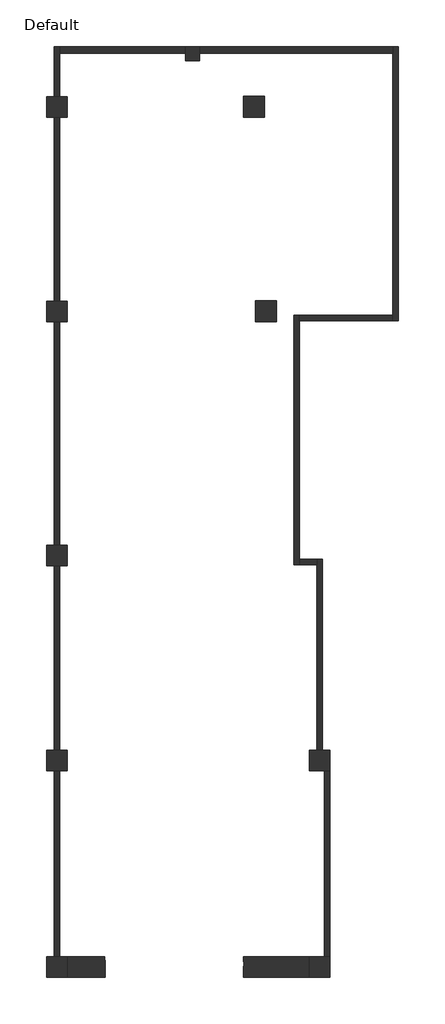
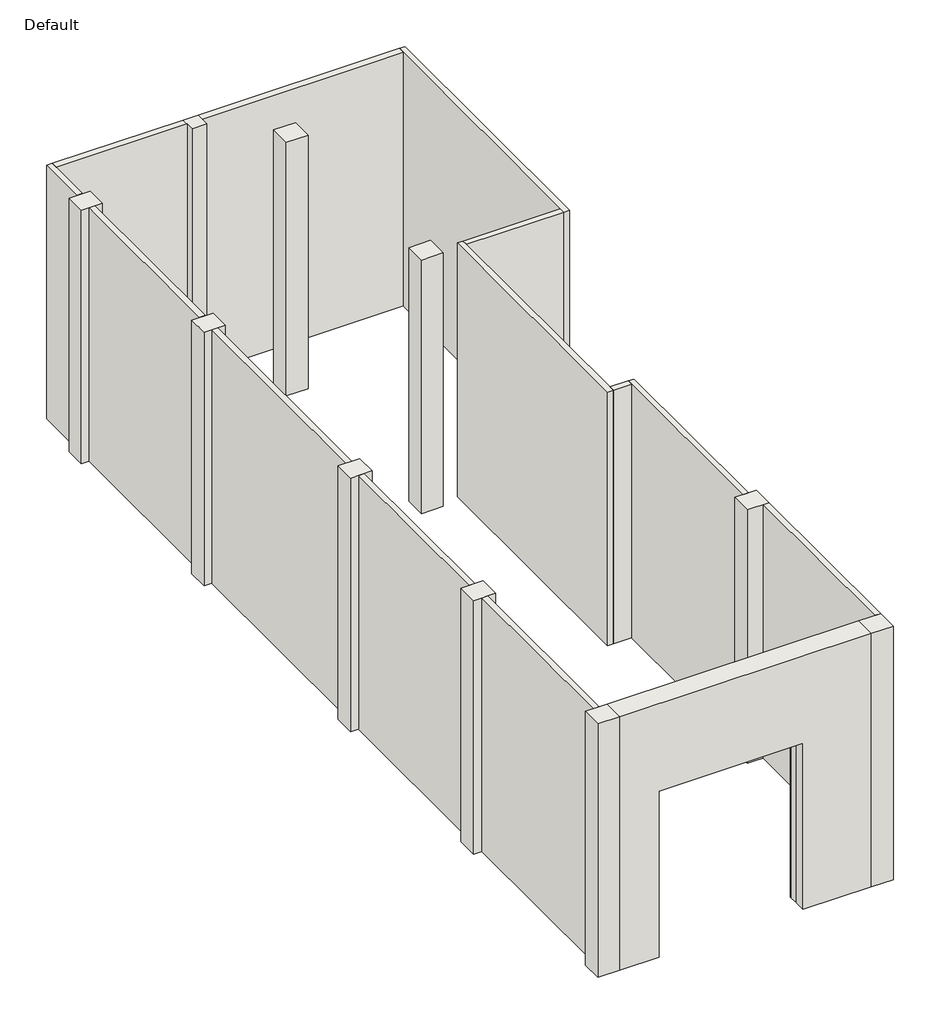
# One storey: 24 walls.
"""IFC4 building model written with IfcOpenShell, lengths in millimetres."""

import ifcopenshell
import ifcopenshell.guid

model = None  # the IFC model being written
_history = None  # IfcOwnerHistory: only IFC2X3 demands one
_inside = {}  # id of a spatial element -> (the spatial element, [elements in it])
_under = {}  # id of a project, library or spatial element -> (it, [spatial elements below it])
_declared = {}  # id of a project -> (the project, [libraries it declares])
_typed = {}  # id of a type object -> (the type object, [elements of that type])
_made_of = {}  # id of a material, layer set ... -> (it, [elements and type objects made of it])


def new_model(schema):
    """Start an empty IFC model of exactly this schema.

    Asked for "IFC4X3", IfcOpenShell would pick the latest addendum, in which some entities
    have other attributes; the version numbers below select the first issue.
    IFC2X3 requires an IfcOwnerHistory on every rooted entity: one is made here for all.
    """
    global model, _history
    if schema == "IFC4X3":
        model = ifcopenshell.file(schema_version=(4, 3, 0, 0))
    else:
        model = ifcopenshell.file(schema=schema)
    _inside.clear()
    _under.clear()
    _declared.clear()
    _typed.clear()
    _made_of.clear()
    _history = None
    if model.schema == "IFC2X3":
        org = make("IfcOrganization", Name="unknown")
        user = make(
            "IfcPersonAndOrganization",
            ThePerson=make("IfcPerson", FamilyName="unknown"),
            TheOrganization=org,
        )
        app = make(
            "IfcApplication",
            ApplicationDeveloper=org,
            Version="unknown",
            ApplicationFullName="unknown",
            ApplicationIdentifier="unknown",
        )
        _history = make(
            "IfcOwnerHistory",
            OwningUser=user,
            OwningApplication=app,
            ChangeAction="ADDED",
            CreationDate=0,
        )
    return model


def make(cls, **values):
    """One entity of the class cls with the attributes given. An attribute that is None is left unset."""
    return model.create_entity(
        cls, **{name: value for name, value in values.items() if value is not None}
    )


def rooted(cls, **values):
    """An entity with a GlobalId (a new one), such as an element, a storey or a relation."""
    return make(cls, GlobalId=ifcopenshell.guid.new(), OwnerHistory=_history, **values)


def si_unit(unit_type, name, prefix=None):
    """IfcSIUnit, for example si_unit("LENGTHUNIT", "METRE", prefix="MILLI")."""
    return make("IfcSIUnit", UnitType=unit_type, Prefix=prefix, Name=name)


def assignment(units):
    """IfcUnitAssignment: the units of a project."""
    return None if units is None else make("IfcUnitAssignment", Units=units)


def point(xyz):
    """IfcCartesianPoint."""
    return None if xyz is None else make("IfcCartesianPoint", Coordinates=xyz)


def direction(xyz):
    """IfcDirection."""
    return None if xyz is None else make("IfcDirection", DirectionRatios=xyz)


def frame(location, z_axis=None, x_axis=None):
    """IfcAxis2Placement3D, a coordinate frame: its origin and axes. An axis left out is left unset."""
    return make(
        "IfcAxis2Placement3D",
        Location=point(location),
        Axis=direction(z_axis),
        RefDirection=direction(x_axis),
    )


def origin():
    """The frame at (0, 0, 0) with its axes left unset."""
    return frame((0.0, 0.0, 0.0))


def origin_with_axes():
    """The frame at (0, 0, 0) with the z axis (0, 0, 1) and the x axis (1, 0, 0) written out."""
    return frame((0.0, 0.0, 0.0), z_axis=(0.0, 0.0, 1.0), x_axis=(1.0, 0.0, 0.0))


def place(relative_to, where):
    """IfcLocalPlacement: puts the frame where relative to a parent placement (None: the world)."""
    return make(
        "IfcLocalPlacement", PlacementRelTo=relative_to, RelativePlacement=where
    )


def context(
    kind, dimensions, precision=None, world=None, true_north=None, identifier=None
):
    """IfcGeometricRepresentationContext, for example the 3D "Model" context."""
    return make(
        "IfcGeometricRepresentationContext",
        ContextIdentifier=identifier,
        ContextType=kind,
        CoordinateSpaceDimension=dimensions,
        Precision=precision,
        WorldCoordinateSystem=world,
        TrueNorth=true_north,
    )


def project(units=None, contexts=None):
    """IfcProject with its units and contexts."""
    return rooted(
        "IfcProject",
        Name="project",
        RepresentationContexts=contexts,
        UnitsInContext=assignment(units),
    )


def spatial(cls, under=None, at=None, **own):
    """A site, building, storey or space (cls), placed at a placement, below another one or the project."""
    s = rooted(cls, ObjectPlacement=at, **own)
    if under is not None:
        _under.setdefault(under.id(), (under, []))[1].append(s)
    return s


def polyline(points):
    """IfcPolyline through the points."""
    return make("IfcPolyline", Points=[point(p) for p in points])


def outline(outer, holes=None, kind="AREA"):
    """IfcArbitraryClosedProfileDef: a profile drawn as a closed curve; with holes, ...WithVoids."""
    if holes is None:
        return make("IfcArbitraryClosedProfileDef", ProfileType=kind, OuterCurve=outer)
    return make(
        "IfcArbitraryProfileDefWithVoids",
        ProfileType=kind,
        OuterCurve=outer,
        InnerCurves=holes,
    )


def extrude(swept, where, along, depth):
    """IfcExtrudedAreaSolid: the profile swept, set in the frame where, extruded along a direction by depth."""
    return make(
        "IfcExtrudedAreaSolid",
        SweptArea=swept,
        Position=where,
        ExtrudedDirection=direction(along),
        Depth=depth,
    )


def faces_of(points, faces, orient=None, outer=None):
    """IfcFace entities. A face is a list of loops; a loop is a list of indices into points, from 0.

    orient and outer hold one flag for each loop. By default every Orientation is true, the
    first loop of a face is its IfcFaceOuterBound and the others are IfcFaceBound.
    """
    made = []
    for i, loops in enumerate(faces):
        bounds = []
        for j, loop in enumerate(loops):
            is_outer = j == 0 if outer is None else outer[i][j]
            bounds.append(
                make(
                    "IfcFaceOuterBound" if is_outer else "IfcFaceBound",
                    Bound=make("IfcPolyLoop", Polygon=[points[k] for k in loop]),
                    Orientation=True if orient is None else orient[i][j],
                )
            )
        made.append(make("IfcFace", Bounds=bounds))
    return made


def faceted_brep(points, faces, orient=None, outer=None, voids=None):
    """IfcFacetedBrep: a solid bounded by flat faces; with voids (closed shells), ...WithVoids."""
    shared = [point(p) for p in points]
    hull = make("IfcClosedShell", CfsFaces=faces_of(shared, faces, orient, outer))
    if voids is None:
        return make("IfcFacetedBrep", Outer=hull)
    return make(
        "IfcFacetedBrepWithVoids",
        Outer=hull,
        Voids=[
            make(cls, CfsFaces=faces_of(shared, fs, o, b)) for cls, fs, o, b in voids
        ],
    )


def shape(context_of_items, identifier, shape_type, items):
    """IfcShapeRepresentation: the items that make up one representation, for example the "Body"."""
    return make(
        "IfcShapeRepresentation",
        ContextOfItems=context_of_items,
        RepresentationIdentifier=identifier,
        RepresentationType=shape_type,
        Items=items,
    )


def source(mapping_origin, context_of_items, identifier, shape_type, items):
    """IfcRepresentationMap: a shape defined once, which mapped items show again and again."""
    return make(
        "IfcRepresentationMap",
        MappingOrigin=mapping_origin,
        MappedRepresentation=shape(context_of_items, identifier, shape_type, items),
    )


def transform(
    local_origin,
    x_axis=None,
    y_axis=None,
    z_axis=None,
    scale=None,
    scale2=None,
    scale3=None,
    uniform=True,
):
    """IfcCartesianTransformationOperator3D, or its non-uniform kind. x_axis, y_axis, z_axis: its Axis1, 2, 3."""
    if uniform:
        return make(
            "IfcCartesianTransformationOperator3D",
            Axis1=direction(x_axis),
            Axis2=direction(y_axis),
            LocalOrigin=point(local_origin),
            Scale=scale,
            Axis3=direction(z_axis),
        )
    return make(
        "IfcCartesianTransformationOperator3DnonUniform",
        Axis1=direction(x_axis),
        Axis2=direction(y_axis),
        LocalOrigin=point(local_origin),
        Scale=scale,
        Axis3=direction(z_axis),
        Scale2=scale2,
        Scale3=scale3,
    )


def mapped(mapping_source, mapping_target):
    """IfcMappedItem: shows the shape of a source again, moved by a transform."""
    return make(
        "IfcMappedItem", MappingSource=mapping_source, MappingTarget=mapping_target
    )


def made_of(thing, what):
    """Note that an element or type object is made of a material, layer set ...; save() writes the relation."""
    if what is not None:
        _made_of.setdefault(what.id(), (what, []))[1].append(thing)
    return thing


def element(
    cls,
    number,
    at=None,
    inside=None,
    cuts=None,
    type_object=None,
    material=None,
    context=None,
    identifier="Body",
    shape_type=None,
    held_by="IfcProductDefinitionShape",
    body=None,
    shapes=None,
    **own,
):
    """One element of the class cls, such as IfcWall. Its Tag is "e" and its number.

    at: its placement. inside: the storey or other place that contains it. cuts: it is an
    opening in that element (IfcRelVoidsElement). A single representation is given by context,
    identifier, shape_type and body (its items); several are given by shapes. held_by: the class
    of the entity that holds the representations. save() writes the other relations.
    """
    e = rooted(cls, Tag="e%d" % number, ObjectPlacement=at, **own)
    if body is not None:
        shapes = [shape(context, identifier, shape_type, body)]
    if shapes is not None:
        e.Representation = make(held_by, Representations=shapes)
    if inside is not None:
        _inside.setdefault(inside.id(), (inside, []))[1].append(e)
    if cuts is not None:
        rooted(
            "IfcRelVoidsElement", RelatingBuildingElement=cuts, RelatedOpeningElement=e
        )
    if type_object is not None:
        _typed.setdefault(type_object.id(), (type_object, []))[1].append(e)
    return made_of(e, material)


def aggregate(whole, parts):
    """IfcRelAggregates: a whole, such as a stair, and the parts it consists of."""
    return rooted("IfcRelAggregates", RelatingObject=whole, RelatedObjects=parts)


def save(model, path):
    """Write the relations noted so far, then the file.

    IfcRelAggregates (storeys below a building ...), IfcRelContainedInSpatialStructure (elements
    in a storey), IfcRelDefinesByType, IfcRelAssociatesMaterial and IfcRelDeclares: one each for
    every whole, place, type object, material and project.
    """
    for whole, parts in _under.values():
        aggregate(whole, parts)
    for where, things in _inside.values():
        rooted(
            "IfcRelContainedInSpatialStructure",
            RelatedElements=things,
            RelatingStructure=where,
        )
    for kind, things in _typed.values():
        rooted("IfcRelDefinesByType", RelatedObjects=things, RelatingType=kind)
    for what, things in _made_of.values():
        rooted("IfcRelAssociatesMaterial", RelatedObjects=things, RelatingMaterial=what)
    for by, libraries in _declared.values():
        rooted("IfcRelDeclares", RelatingContext=by, RelatedDefinitions=libraries)
    model.write(path)


def pillar_1_pillar_1_f30ecb4e(model_context):
    return source(origin(), model_context, "Body", "SweptSolid", [
        extrude(outline(polyline([(240.0, 0.0), (-140.0, 0.0), (-140.0, 380.0), (240.0, 380.0), (240.0, 0.0)])), origin_with_axes(), (0.0, 0.0, 1.0), 4700.0),
    ])


def pillar_10_pillar_10_9a1170d5(model_context):
    return source(origin(), model_context, "Body", "SweptSolid", [
        extrude(outline(polyline([(5040.0, 0.0), (4660.0, 0.0), (4660.0, 380.0), (5040.0, 380.0), (5040.0, 0.0)])), origin_with_axes(), (0.0, 0.0, 1.0), 4700.0),
    ])


def pillar_2_pillar_2_c342d97b(model_context):
    return source(origin(), model_context, "Body", "SweptSolid", [
        extrude(outline(polyline([(240.0, 3770.0), (-140.0, 3770.0), (-140.0, 4150.0), (240.0, 4150.0), (240.0, 3770.0)])), origin_with_axes(), (0.0, 0.0, 1.0), 4700.0),
    ])


def pillar_3_pillar_3_bef34371(model_context):
    return source(origin(), model_context, "Body", "SweptSolid", [
        extrude(outline(polyline([(240.0, 7510.0), (-140.0, 7510.0), (-140.0, 7890.0), (240.0, 7890.0), (240.0, 7510.0)])), origin_with_axes(), (0.0, 0.0, 1.0), 4700.0),
    ])


def pillar_4_pillar_4_1424975a(model_context):
    return source(origin(), model_context, "Body", "SweptSolid", [
        extrude(outline(polyline([(235.0, 11970.0), (-135.0, 11970.0), (-135.0, 12340.0), (235.0, 12340.0), (235.0, 11970.0)])), origin_with_axes(), (0.0, 0.0, 1.0), 4700.0),
    ])


def pillar_5_pillar_5_5ba1b83c(model_context):
    return source(origin(), model_context, "Body", "SweptSolid", [
        extrude(outline(polyline([(235.0, 15700.0), (-135.0, 15700.0), (-135.0, 16070.0), (235.0, 16070.0), (235.0, 15700.0)])), origin_with_axes(), (0.0, 0.0, 1.0), 4700.0),
    ])


def pillar_6_pillar_6_704e6477(model_context):
    return source(origin(), model_context, "Body", "SweptSolid", [
        extrude(outline(polyline([(2660.0, 16730.0), (2400.0, 16730.0), (2400.0, 16990.0), (2660.0, 16990.0), (2660.0, 16730.0)])), origin_with_axes(), (0.0, 0.0, 1.0), 4700.0),
    ])


def pillar_7_pillar_7_9e6fd231(model_context):
    return source(origin(), model_context, "Body", "SweptSolid", [
        extrude(outline(polyline([(3840.0, 15700.0), (3460.0, 15700.0), (3460.0, 16080.0), (3840.0, 16080.0), (3840.0, 15700.0)])), origin_with_axes(), (0.0, 0.0, 1.0), 4700.0),
    ])


def pillar_8_pillar_8_cf5ea2e7(model_context):
    return source(origin(), model_context, "Body", "SweptSolid", [
        extrude(outline(polyline([(4060.0, 11970.0), (3680.0, 11970.0), (3680.0, 12350.0), (4060.0, 12350.0), (4060.0, 11970.0)])), origin_with_axes(), (0.0, 0.0, 1.0), 4700.0),
    ])


def pillar_9_pillar_9_1ccd6465(model_context):
    return source(origin(), model_context, "Body", "SweptSolid", [
        extrude(outline(polyline([(5040.0, 3770.0), (4660.0, 3770.0), (4660.0, 4150.0), (5040.0, 4150.0), (5040.0, 3770.0)])), origin_with_axes(), (0.0, 0.0, 1.0), 4700.0),
    ])


def wall_1_wall_1_841e26ce(model_context):
    return source(origin(), model_context, "Body", "SweptSolid", [
        extrude(outline(polyline([(100.0, 3770.0), (100.0, 380.0), (0.0, 380.0), (0.0, 3770.0), (100.0, 3770.0)])), origin_with_axes(), (0.0, 0.0, 1.0), 4700.0),
    ])


def wall_10_wall_10_bc7aa466(model_context):
    return source(origin(), model_context, "Body", "SweptSolid", [
        extrude(outline(polyline([(4480.0, 12090.0), (4480.0, 7530.0), (4380.0, 7530.0), (4380.0, 12090.0), (4480.0, 12090.0)])), origin_with_axes(), (0.0, 0.0, 1.0), 4700.0),
    ])


def wall_11_wall_11_b3d456f5(model_context):
    return source(origin(), model_context, "Body", "SweptSolid", [
        extrude(outline(polyline([(4800.0, 7530.0), (4480.0, 7530.0), (4480.0, 7630.0), (4800.0, 7630.0), (4800.0, 7530.0)])), origin_with_axes(), (0.0, 0.0, 1.0), 4700.0),
    ])


def wall_12_wall_12_6134a25a(model_context):
    return source(origin(), model_context, "Body", "SweptSolid", [
        extrude(outline(polyline([(4900.0, 7630.0), (4900.0, 4150.0), (4800.0, 4150.0), (4800.0, 7630.0), (4900.0, 7630.0)])), origin_with_axes(), (0.0, 0.0, 1.0), 4700.0),
    ])


def wall_13_wall_13_25ff5e73(model_context):
    return source(origin(), model_context, "Body", "SweptSolid", [
        extrude(outline(polyline([(5040.0, 3770.0), (5040.0, 380.0), (4940.0, 380.0), (4940.0, 3770.0), (5040.0, 3770.0)])), origin_with_axes(), (0.0, 0.0, 1.0), 4700.0),
    ])


def wall_14_wall_14_043e5d1d(model_context):
    return source(origin(), model_context, "Body", "Brep", [
        faceted_brep([(4660.0, 0.0, 4700.0), (4660.0, 380.0, 4700.0), (240.0, 380.0, 4700.0), (240.0, 0.0, 4700.0), (240.0, 0.0, 0.0), (240.0, 380.0, 0.0), (926.5217391, 380.0, 0.0), (930.0, 270.0, 0.0), (930.0, 0.0, 0.0), (4660.0, 380.0, 0.0), (4660.0, 0.0, 0.0), (3460.0, 0.0, 0.0), (3460.0, 199.9250293, 0.0), (3464.7407136, 200.0749333, 0.0), (3460.0, 350.0, 0.0), (3460.0, 380.0, 0.0), (3460.0, 380.0, 3080.0), (3459.0513834, 380.0, 3080.0), (3459.0513834, 380.0, 4050.0), (926.5217391, 380.0, 4050.0), (930.0, 0.0, 3080.0), (3460.0, 0.0, 3080.0), (3464.7407136, 200.0749333, 4050.0), (934.7407136, 120.0749333, 4050.0), (3460.0, 350.0, 3080.0), (934.7407136, 120.0749333, 3080.0), (930.0, 270.0, 3080.0), (3460.0, 199.9250293, 3080.0)], [[[0, 1, 2, 3]], [[4, 5, 6, 7, 8]], [[9, 10, 11, 12, 13, 14, 15]], [[1, 0, 10, 9]], [[2, 1, 9, 15, 16, 17, 18, 19, 6, 5]], [[3, 2, 5, 4]], [[0, 3, 4, 8, 20, 21, 11, 10]], [[22, 23, 19, 18]], [[13, 22, 18, 17, 24, 14]], [[19, 23, 25, 26, 7, 6]], [[23, 22, 13, 12, 27, 25]], [[20, 26, 25, 27, 21]], [[16, 24, 17]], [[21, 27, 12, 11]], [[24, 16, 15, 14]], [[26, 20, 8, 7]]]),
    ])


def wall_2_wall_2_345a8b54(model_context):
    return source(origin(), model_context, "Body", "SweptSolid", [
        extrude(outline(polyline([(100.0, 7510.0), (100.0, 4150.0), (0.0, 4150.0), (0.0, 7510.0), (100.0, 7510.0)])), origin_with_axes(), (0.0, 0.0, 1.0), 4700.0),
    ])


def wall_3_wall_3_2bae312e(model_context):
    return source(origin(), model_context, "Body", "SweptSolid", [
        extrude(outline(polyline([(100.0, 11970.0), (100.0, 7890.0), (0.0, 7890.0), (0.0, 11970.0), (100.0, 11970.0)])), origin_with_axes(), (0.0, 0.0, 1.0), 4700.0),
    ])


def wall_4_wall_4_e46e00ff(model_context):
    return source(origin(), model_context, "Body", "SweptSolid", [
        extrude(outline(polyline([(100.0, 15700.0), (100.0, 12350.0), (0.0, 12350.0), (0.0, 15700.0), (100.0, 15700.0)])), origin_with_axes(), (0.0, 0.0, 1.0), 4700.0),
    ])


def wall_5_wall_5_558b8a57(model_context):
    return source(origin(), model_context, "Body", "SweptSolid", [
        extrude(outline(polyline([(100.0, 16990.0), (100.0, 16080.0), (0.0, 16080.0), (0.0, 16990.0), (100.0, 16990.0)])), origin_with_axes(), (0.0, 0.0, 1.0), 4700.0),
    ])


def wall_6_wall_6_c3d1f71e(model_context):
    return source(origin(), model_context, "Body", "SweptSolid", [
        extrude(outline(polyline([(2400.0, 16870.0), (100.0, 16870.0), (100.0, 16990.0), (2400.0, 16990.0), (2400.0, 16870.0)])), origin_with_axes(), (0.0, 0.0, 1.0), 4700.0),
    ])


def wall_7_wall_7_843a4671(model_context):
    return source(origin(), model_context, "Body", "SweptSolid", [
        extrude(outline(polyline([(6190.0, 16870.0), (2660.0, 16870.0), (2660.0, 16990.0), (6190.0, 16990.0), (6190.0, 16870.0)])), origin_with_axes(), (0.0, 0.0, 1.0), 4700.0),
    ])


def wall_8_wall_8_015fc5ca(model_context):
    return source(origin(), model_context, "Body", "SweptSolid", [
        extrude(outline(polyline([(6290.0, 16990.0), (6290.0, 11990.0), (6190.0, 11990.0), (6190.0, 16990.0), (6290.0, 16990.0)])), origin_with_axes(), (0.0, 0.0, 1.0), 4700.0),
    ])


def wall_9_wall_9_7e9080d3(model_context):
    return source(origin(), model_context, "Body", "SweptSolid", [
        extrude(outline(polyline([(6190.0, 11990.0), (4480.0, 11990.0), (4480.0, 12090.0), (6190.0, 12090.0), (6190.0, 11990.0)])), origin_with_axes(), (0.0, 0.0, 1.0), 4700.0),
    ])


model = new_model("IFC4")

# Units and contexts
model_context = context("Model", 3, world=origin())
ifc_project = project(units=[si_unit("LENGTHUNIT", "METRE", prefix="MILLI")], contexts=[model_context])

# Site, building, storey
site = spatial("IfcSite", under=ifc_project)
building = spatial("IfcBuilding", under=site)
storey = spatial("IfcBuildingStorey", under=building, Name="Default", Elevation=0.0)

# Walls
placement = place(None, origin())
pillar_1_pillar_1_shape = pillar_1_pillar_1_f30ecb4e(model_context)
element("IfcWall", 1, ObjectType="Pillar_1 : Pillar_1", at=placement, inside=storey, context=model_context, shape_type="MappedRepresentation", body=[
    mapped(pillar_1_pillar_1_shape, transform((0.0, 0.0, 0.0), x_axis=(1.0, 0.0, 0.0), y_axis=(0.0, 1.0, 0.0), z_axis=(0.0, 0.0, 1.0))),
])
pillar_10_pillar_10_shape = pillar_10_pillar_10_9a1170d5(model_context)
element("IfcWall", 2, ObjectType="Pillar_10 : Pillar_10", at=placement, inside=storey, context=model_context, shape_type="MappedRepresentation", body=[
    mapped(pillar_10_pillar_10_shape, transform((0.0, 0.0, 0.0), x_axis=(1.0, 0.0, 0.0), y_axis=(0.0, 1.0, 0.0), z_axis=(0.0, 0.0, 1.0))),
])
pillar_2_pillar_2_shape = pillar_2_pillar_2_c342d97b(model_context)
element("IfcWall", 3, ObjectType="Pillar_2 : Pillar_2", at=placement, inside=storey, context=model_context, shape_type="MappedRepresentation", body=[
    mapped(pillar_2_pillar_2_shape, transform((0.0, 0.0, 0.0), x_axis=(1.0, 0.0, 0.0), y_axis=(0.0, 1.0, 0.0), z_axis=(0.0, 0.0, 1.0))),
])
pillar_3_pillar_3_shape = pillar_3_pillar_3_bef34371(model_context)
element("IfcWall", 4, ObjectType="Pillar_3 : Pillar_3", at=placement, inside=storey, context=model_context, shape_type="MappedRepresentation", body=[
    mapped(pillar_3_pillar_3_shape, transform((0.0, 0.0, 0.0), x_axis=(1.0, 0.0, 0.0), y_axis=(0.0, 1.0, 0.0), z_axis=(0.0, 0.0, 1.0))),
])
pillar_4_pillar_4_shape = pillar_4_pillar_4_1424975a(model_context)
element("IfcWall", 5, ObjectType="Pillar_4 : Pillar_4", at=placement, inside=storey, context=model_context, shape_type="MappedRepresentation", body=[
    mapped(pillar_4_pillar_4_shape, transform((0.0, 0.0, 0.0), x_axis=(1.0, 0.0, 0.0), y_axis=(0.0, 1.0, 0.0), z_axis=(0.0, 0.0, 1.0))),
])
pillar_5_pillar_5_shape = pillar_5_pillar_5_5ba1b83c(model_context)
element("IfcWall", 6, ObjectType="Pillar_5 : Pillar_5", at=placement, inside=storey, context=model_context, shape_type="MappedRepresentation", body=[
    mapped(pillar_5_pillar_5_shape, transform((0.0, 0.0, 0.0), x_axis=(1.0, 0.0, 0.0), y_axis=(0.0, 1.0, 0.0), z_axis=(0.0, 0.0, 1.0))),
])
pillar_6_pillar_6_shape = pillar_6_pillar_6_704e6477(model_context)
element("IfcWall", 7, ObjectType="Pillar_6 : Pillar_6", at=placement, inside=storey, context=model_context, shape_type="MappedRepresentation", body=[
    mapped(pillar_6_pillar_6_shape, transform((0.0, 0.0, 0.0), x_axis=(1.0, 0.0, 0.0), y_axis=(0.0, 1.0, 0.0), z_axis=(0.0, 0.0, 1.0))),
])
pillar_7_pillar_7_shape = pillar_7_pillar_7_9e6fd231(model_context)
element("IfcWall", 8, ObjectType="Pillar_7 : Pillar_7", at=placement, inside=storey, context=model_context, shape_type="MappedRepresentation", body=[
    mapped(pillar_7_pillar_7_shape, transform((0.0, 0.0, 0.0), x_axis=(1.0, 0.0, 0.0), y_axis=(0.0, 1.0, 0.0), z_axis=(0.0, 0.0, 1.0))),
])
pillar_8_pillar_8_shape = pillar_8_pillar_8_cf5ea2e7(model_context)
element("IfcWall", 9, ObjectType="Pillar_8 : Pillar_8", at=placement, inside=storey, context=model_context, shape_type="MappedRepresentation", body=[
    mapped(pillar_8_pillar_8_shape, transform((0.0, 0.0, 0.0), x_axis=(1.0, 0.0, 0.0), y_axis=(0.0, 1.0, 0.0), z_axis=(0.0, 0.0, 1.0))),
])
pillar_9_pillar_9_shape = pillar_9_pillar_9_1ccd6465(model_context)
element("IfcWall", 10, ObjectType="Pillar_9 : Pillar_9", at=placement, inside=storey, context=model_context, shape_type="MappedRepresentation", body=[
    mapped(pillar_9_pillar_9_shape, transform((0.0, 0.0, 0.0), x_axis=(1.0, 0.0, 0.0), y_axis=(0.0, 1.0, 0.0), z_axis=(0.0, 0.0, 1.0))),
])
wall_1_wall_1_shape = wall_1_wall_1_841e26ce(model_context)
element("IfcWall", 11, ObjectType="Wall_1 : Wall_1", at=placement, inside=storey, context=model_context, shape_type="MappedRepresentation", body=[
    mapped(wall_1_wall_1_shape, transform((0.0, 0.0, 0.0), x_axis=(1.0, 0.0, 0.0), y_axis=(0.0, 1.0, 0.0), z_axis=(0.0, 0.0, 1.0))),
])
wall_10_wall_10_shape = wall_10_wall_10_bc7aa466(model_context)
element("IfcWall", 12, ObjectType="Wall_10 : Wall_10", at=placement, inside=storey, context=model_context, shape_type="MappedRepresentation", body=[
    mapped(wall_10_wall_10_shape, transform((0.0, 0.0, 0.0), x_axis=(1.0, 0.0, 0.0), y_axis=(0.0, 1.0, 0.0), z_axis=(0.0, 0.0, 1.0))),
])
wall_11_wall_11_shape = wall_11_wall_11_b3d456f5(model_context)
element("IfcWall", 13, ObjectType="Wall_11 : Wall_11", at=placement, inside=storey, context=model_context, shape_type="MappedRepresentation", body=[
    mapped(wall_11_wall_11_shape, transform((0.0, 0.0, 0.0), x_axis=(1.0, 0.0, 0.0), y_axis=(0.0, 1.0, 0.0), z_axis=(0.0, 0.0, 1.0))),
])
wall_12_wall_12_shape = wall_12_wall_12_6134a25a(model_context)
element("IfcWall", 14, ObjectType="Wall_12 : Wall_12", at=placement, inside=storey, context=model_context, shape_type="MappedRepresentation", body=[
    mapped(wall_12_wall_12_shape, transform((0.0, 0.0, 0.0), x_axis=(1.0, 0.0, 0.0), y_axis=(0.0, 1.0, 0.0), z_axis=(0.0, 0.0, 1.0))),
])
wall_13_wall_13_shape = wall_13_wall_13_25ff5e73(model_context)
element("IfcWall", 15, ObjectType="Wall_13 : Wall_13", at=placement, inside=storey, context=model_context, shape_type="MappedRepresentation", body=[
    mapped(wall_13_wall_13_shape, transform((0.0, 0.0, 0.0), x_axis=(1.0, 0.0, 0.0), y_axis=(0.0, 1.0, 0.0), z_axis=(0.0, 0.0, 1.0))),
])
wall_14_wall_14_shape = wall_14_wall_14_043e5d1d(model_context)
element("IfcWall", 16, ObjectType="Wall_14 : Wall_14", at=placement, inside=storey, context=model_context, shape_type="MappedRepresentation", body=[
    mapped(wall_14_wall_14_shape, transform((0.0, 0.0, 0.0), x_axis=(1.0, 0.0, 0.0), y_axis=(0.0, 1.0, 0.0), z_axis=(0.0, 0.0, 1.0))),
])
wall_2_wall_2_shape = wall_2_wall_2_345a8b54(model_context)
element("IfcWall", 17, ObjectType="Wall_2 : Wall_2", at=placement, inside=storey, context=model_context, shape_type="MappedRepresentation", body=[
    mapped(wall_2_wall_2_shape, transform((0.0, 0.0, 0.0), x_axis=(1.0, 0.0, 0.0), y_axis=(0.0, 1.0, 0.0), z_axis=(0.0, 0.0, 1.0))),
])
wall_3_wall_3_shape = wall_3_wall_3_2bae312e(model_context)
element("IfcWall", 18, ObjectType="Wall_3 : Wall_3", at=placement, inside=storey, context=model_context, shape_type="MappedRepresentation", body=[
    mapped(wall_3_wall_3_shape, transform((0.0, 0.0, 0.0), x_axis=(1.0, 0.0, 0.0), y_axis=(0.0, 1.0, 0.0), z_axis=(0.0, 0.0, 1.0))),
])
wall_4_wall_4_shape = wall_4_wall_4_e46e00ff(model_context)
element("IfcWall", 19, ObjectType="Wall_4 : Wall_4", at=placement, inside=storey, context=model_context, shape_type="MappedRepresentation", body=[
    mapped(wall_4_wall_4_shape, transform((0.0, 0.0, 0.0), x_axis=(1.0, 0.0, 0.0), y_axis=(0.0, 1.0, 0.0), z_axis=(0.0, 0.0, 1.0))),
])
wall_5_wall_5_shape = wall_5_wall_5_558b8a57(model_context)
element("IfcWall", 20, ObjectType="Wall_5 : Wall_5", at=placement, inside=storey, context=model_context, shape_type="MappedRepresentation", body=[
    mapped(wall_5_wall_5_shape, transform((0.0, 0.0, 0.0), x_axis=(1.0, 0.0, 0.0), y_axis=(0.0, 1.0, 0.0), z_axis=(0.0, 0.0, 1.0))),
])
wall_6_wall_6_shape = wall_6_wall_6_c3d1f71e(model_context)
element("IfcWall", 21, ObjectType="Wall_6 : Wall_6", at=placement, inside=storey, context=model_context, shape_type="MappedRepresentation", body=[
    mapped(wall_6_wall_6_shape, transform((0.0, 0.0, 0.0), x_axis=(1.0, 0.0, 0.0), y_axis=(0.0, 1.0, 0.0), z_axis=(0.0, 0.0, 1.0))),
])
wall_7_wall_7_shape = wall_7_wall_7_843a4671(model_context)
element("IfcWall", 22, ObjectType="Wall_7 : Wall_7", at=placement, inside=storey, context=model_context, shape_type="MappedRepresentation", body=[
    mapped(wall_7_wall_7_shape, transform((0.0, 0.0, 0.0), x_axis=(1.0, 0.0, 0.0), y_axis=(0.0, 1.0, 0.0), z_axis=(0.0, 0.0, 1.0))),
])
wall_8_wall_8_shape = wall_8_wall_8_015fc5ca(model_context)
element("IfcWall", 23, ObjectType="Wall_8 : Wall_8", at=placement, inside=storey, context=model_context, shape_type="MappedRepresentation", body=[
    mapped(wall_8_wall_8_shape, transform((0.0, 0.0, 0.0), x_axis=(1.0, 0.0, 0.0), y_axis=(0.0, 1.0, 0.0), z_axis=(0.0, 0.0, 1.0))),
])
wall_9_wall_9_shape = wall_9_wall_9_7e9080d3(model_context)
element("IfcWall", 24, ObjectType="Wall_9 : Wall_9", at=placement, inside=storey, context=model_context, shape_type="MappedRepresentation", body=[
    mapped(wall_9_wall_9_shape, transform((0.0, 0.0, 0.0), x_axis=(1.0, 0.0, 0.0), y_axis=(0.0, 1.0, 0.0), z_axis=(0.0, 0.0, 1.0))),
])

save(model, "model.ifc")

# Revit data of these elements
# Project information
#   IfcApplicationVersion = "0.19 build 24366 (Git)"
#   IfcApplicationName = "FreeCAD"
#   IfcBuilding GUID = "1g_7ni_KL3awAxLE_935$K"
#   IfcProject GUID = "37f9L3Jlz9hgw3PJK84Ga4"
#   NameOverride = "Default Building"
#   Project Issue Date = "Issue Date"
#   Project Status = "Project Status"
#   Client Name = "Owner"
#   Project Address = "Enter address here"
#   Project Name = "Project Name"
#   Project Number = "Project Number"
# Type "Pillar_1 : Pillar_1"
#   NameOverride = "Pillar_1"
# Type "Pillar_10 : Pillar_10"
#   NameOverride = "Pillar_10"
# Type "Pillar_2 : Pillar_2"
#   NameOverride = "Pillar_2"
# Type "Pillar_3 : Pillar_3"
#   NameOverride = "Pillar_3"
# Type "Pillar_4 : Pillar_4"
#   NameOverride = "Pillar_4"
# Type "Pillar_5 : Pillar_5"
#   NameOverride = "Pillar_5"
# Type "Pillar_6 : Pillar_6"
#   NameOverride = "Pillar_6"
# Type "Pillar_7 : Pillar_7"
#   NameOverride = "Pillar_7"
# Type "Pillar_8 : Pillar_8"
#   NameOverride = "Pillar_8"
# Type "Pillar_9 : Pillar_9"
#   NameOverride = "Pillar_9"
# Type "Wall_1 : Wall_1"
#   NameOverride = "Wall_1"
# Type "Wall_10 : Wall_10"
#   NameOverride = "Wall_10"
# Type "Wall_11 : Wall_11"
#   NameOverride = "Wall_11"
# Type "Wall_12 : Wall_12"
#   NameOverride = "Wall_12"
# Type "Wall_13 : Wall_13"
#   NameOverride = "Wall_13"
# Type "Wall_14 : Wall_14"
#   NameOverride = "Wall_14"
# Type "Wall_2 : Wall_2"
#   NameOverride = "Wall_2"
# Type "Wall_3 : Wall_3"
#   NameOverride = "Wall_3"
# Type "Wall_4 : Wall_4"
#   NameOverride = "Wall_4"
# Type "Wall_5 : Wall_5"
#   NameOverride = "Wall_5"
# Type "Wall_6 : Wall_6"
#   NameOverride = "Wall_6"
# Type "Wall_7 : Wall_7"
#   NameOverride = "Wall_7"
# Type "Wall_8 : Wall_8"
#   NameOverride = "Wall_8"
# Type "Wall_9 : Wall_9"
#   NameOverride = "Wall_9"
# Element 1 (IfcWall, "Pillar_1 : Pillar_1")
#   IfcGUID = "0i3U4bonrFQuLvhPGY5Gun"
#   Phase Created = New Construction
#   Materials on its faces: "IfcSurfaceStyle #33"
# Element 2 (IfcWall, "Pillar_10 : Pillar_10")
#   IfcGUID = "1jV9h38mX0HQYQoqGTi02u"
#   Phase Created = New Construction
#   Materials on its faces: "IfcSurfaceStyle #33"
# Element 3 (IfcWall, "Pillar_2 : Pillar_2")
#   IfcGUID = "2JmMf2RTXDIx0NJJb3MlgR"
#   Phase Created = New Construction
#   Materials on its faces: "IfcSurfaceStyle #33"
# Element 4 (IfcWall, "Pillar_3 : Pillar_3")
#   IfcGUID = "2RQwCSCpD3FxNyQ6eLRzV0"
#   Phase Created = New Construction
#   Materials on its faces: "IfcSurfaceStyle #33"
# Element 5 (IfcWall, "Pillar_4 : Pillar_4")
#   IfcGUID = "2oplVHAEfDRQDOu$GeLT_e"
#   Phase Created = New Construction
#   Materials on its faces: "IfcSurfaceStyle #33"
# Element 6 (IfcWall, "Pillar_5 : Pillar_5")
#   IfcGUID = "374hwgaifA6A9KN0wtLfkG"
#   Phase Created = New Construction
#   Materials on its faces: "IfcSurfaceStyle #33"
# Element 7 (IfcWall, "Pillar_6 : Pillar_6")
#   IfcGUID = "3wBRFIdmP88BAmNX6$w8k4"
#   Phase Created = New Construction
#   Materials on its faces: "IfcSurfaceStyle #33"
# Element 8 (IfcWall, "Pillar_7 : Pillar_7")
#   IfcGUID = "1rNhQaMNr3sg79PVHFGGkv"
#   Phase Created = New Construction
#   Materials on its faces: "IfcSurfaceStyle #33"
# Element 9 (IfcWall, "Pillar_8 : Pillar_8")
#   IfcGUID = "34PfvF90j6gP2I5_G2$Aod"
#   Phase Created = New Construction
#   Materials on its faces: "IfcSurfaceStyle #33"
# Element 10 (IfcWall, "Pillar_9 : Pillar_9")
#   IfcGUID = "1tCiwBhXn9H8H8WP08qlOy"
#   Phase Created = New Construction
#   Materials on its faces: "IfcSurfaceStyle #33"
# Element 11 (IfcWall, "Wall_1 : Wall_1")
#   IfcGUID = "3rC2uzHqHE3Ow2uRGFsTXP"
#   Phase Created = New Construction
#   Materials on its faces: "IfcSurfaceStyle #33"
# Element 12 (IfcWall, "Wall_10 : Wall_10")
#   IfcGUID = "1z2KDPPa15k8V3KVZtnNoy"
#   Phase Created = New Construction
#   Materials on its faces: "IfcSurfaceStyle #33"
# Element 13 (IfcWall, "Wall_11 : Wall_11")
#   IfcGUID = "3AVe2MIAv5fhFacUUvOx_U"
#   Phase Created = New Construction
#   Materials on its faces: "IfcSurfaceStyle #33"
# Element 14 (IfcWall, "Wall_12 : Wall_12")
#   IfcGUID = "1Urq34tlTF_wC29zH6wIWX"
#   Phase Created = New Construction
#   Materials on its faces: "IfcSurfaceStyle #33"
# Element 15 (IfcWall, "Wall_13 : Wall_13")
#   IfcGUID = "3R$HgMJ6HB2PNeWNls0K1x"
#   Phase Created = New Construction
#   Materials on its faces: "IfcSurfaceStyle #33"
# Element 16 (IfcWall, "Wall_14 : Wall_14")
#   IfcGUID = "1ubvNAZ8PCi9v0QtSpMAc4"
#   Phase Created = New Construction
#   Materials on its faces: "IfcSurfaceStyle #33"
# Element 17 (IfcWall, "Wall_2 : Wall_2")
#   IfcGUID = "0QlNCus9TAf9J_Qzb2UqET"
#   Phase Created = New Construction
#   Materials on its faces: "IfcSurfaceStyle #33"
# Element 18 (IfcWall, "Wall_3 : Wall_3")
#   IfcGUID = "0bbAE_YY5EWeVhuP51kTyS"
#   Phase Created = New Construction
#   Materials on its faces: "IfcSurfaceStyle #33"
# Element 19 (IfcWall, "Wall_4 : Wall_4")
#   IfcGUID = "2fZ5c6am1FGvykYZYI20ah"
#   Phase Created = New Construction
#   Materials on its faces: "IfcSurfaceStyle #33"
# Element 20 (IfcWall, "Wall_5 : Wall_5")
#   IfcGUID = "2$ipg7paHFuRssTHWcTQwP"
#   Phase Created = New Construction
#   Materials on its faces: "IfcSurfaceStyle #33"
# Element 21 (IfcWall, "Wall_6 : Wall_6")
#   IfcGUID = "19QYy1k8j7M8MfbHl17fx0"
#   Phase Created = New Construction
#   Materials on its faces: "IfcSurfaceStyle #33"
# Element 22 (IfcWall, "Wall_7 : Wall_7")
#   IfcGUID = "2l8vKaR0H5SvXrs92HfGs_"
#   Phase Created = New Construction
#   Materials on its faces: "IfcSurfaceStyle #33"
# Element 23 (IfcWall, "Wall_8 : Wall_8")
#   IfcGUID = "2Qmf7Qr0bASh4FCcVHQ80M"
#   Phase Created = New Construction
#   Materials on its faces: "IfcSurfaceStyle #33"
# Element 24 (IfcWall, "Wall_9 : Wall_9")
#   IfcGUID = "3SoRaDAT93Pg2TcdourkZ2"
#   Phase Created = New Construction
#   Materials on its faces: "IfcSurfaceStyle #33"
# Materials
#   "IfcSurfaceStyle #33": class "Unassigned", colour RGB 214 214 214, transparency 0
